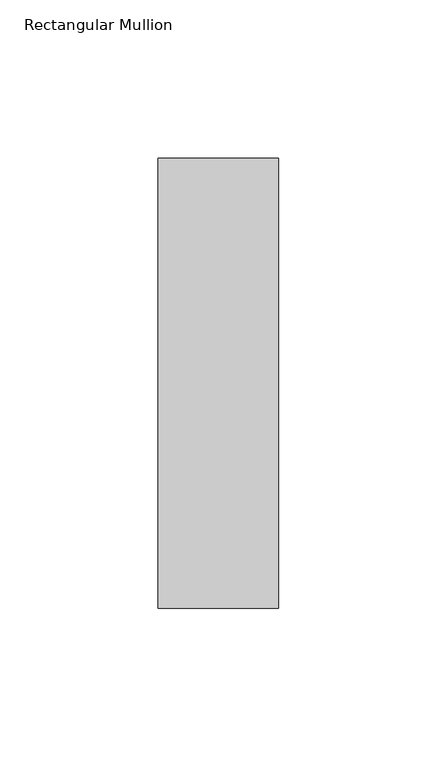
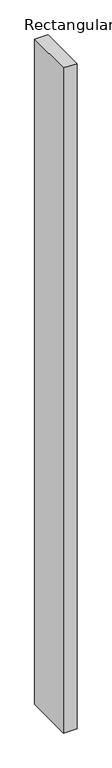
"""IFC4 building model written with IfcOpenShell, lengths in millimetres: member geometry, Rectangular Mullion : NLRS_21_CWM_hsb-regel 38x142_gen_rsf."""

from ifc_helpers import new_model, si_unit, frame, origin, place, context, project, spatial, polyline, outline, extrude, source, transform, mapped, element, save


def rectangular_mullion_a27e35f8(model_context):
    return source(origin(), model_context, "Body", "SweptSolid", [
        extrude(outline(polyline([(19.0, -71.0), (-19.0, -71.0), (-19.0, 71.0), (19.0, 71.0), (19.0, -71.0)])), frame((0.0, 0.0, -2000.0), z_axis=(0.0, 0.0, 1.0), x_axis=(1.0, 0.0, 0.0)), (0.0, 0.0, 1.0), 2000.0),
    ])


if __name__ == "__main__":
    model = new_model("IFC4")
    model_context = context("Model", 3, world=origin())
    ifc_project = project(units=[si_unit("LENGTHUNIT", "METRE", prefix="MILLI")], contexts=[model_context])
    site = spatial("IfcSite", under=ifc_project)
    building = spatial("IfcBuilding", under=site)
    placement = place(None, origin())
    rectangular_mullion_shape = rectangular_mullion_a27e35f8(model_context)
    element("IfcMember", 1, ObjectType="Rectangular Mullion : NLRS_21_CWM_hsb-regel 38x142_gen_rsf", at=placement, inside=building, context=model_context, shape_type="MappedRepresentation", body=[
        mapped(rectangular_mullion_shape, transform((0.0, 0.0, 0.0), x_axis=(1.0, 0.0, 0.0), y_axis=(0.0, 1.0, 0.0), z_axis=(0.0, 0.0, 1.0))),
    ])
    save(model, "model.ifc")

# Revit data of these elements
# Type "Rectangular Mullion : NLRS_21_CWM_hsb-regel 38x142_gen_rsf"
#   Export Type to IFC As = "IfcWall"
#   Type IfcGUID = "07M7mRoiH1CR8m_RSKIwpF"
#   Assembly Code = "21.10"
#   built-in parameter 1007322 = 0.465879 (stored number, unit not read)
#   built-in parameter 1007321 = 0.062336 (stored number, unit not read)
#   built-in parameter 1007320 = 0.062336 (stored number, unit not read)
# Element 1 (IfcMember, "Rectangular Mullion : NLRS_21_CWM_hsb-regel 38x142_gen_rsf")
#   Materials on its faces: "NLRS_i2_hout naaldhout vuren_gen_rsf"
# Materials
#   "NLRS_i2_hout naaldhout vuren_gen_rsf": class "I - Hout", colour RGB 234 199 147, transparency 0, Keynote = "i2", Manufacturer = "Revit Standards Foundation", URL = "www.revitstandards.org", Description = "hout vuren", Cost = 0
